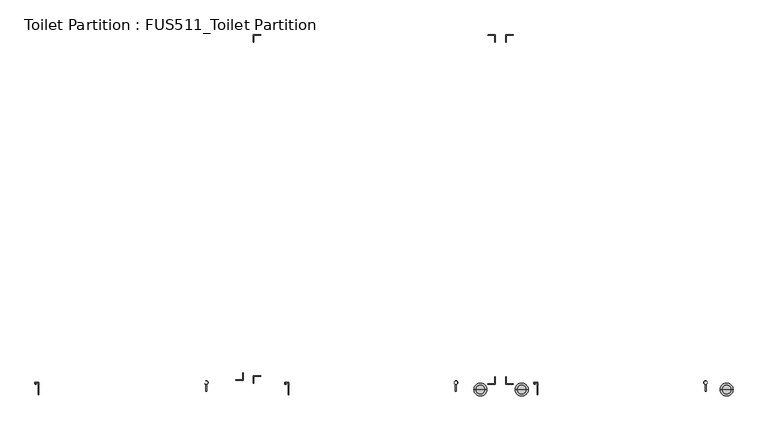
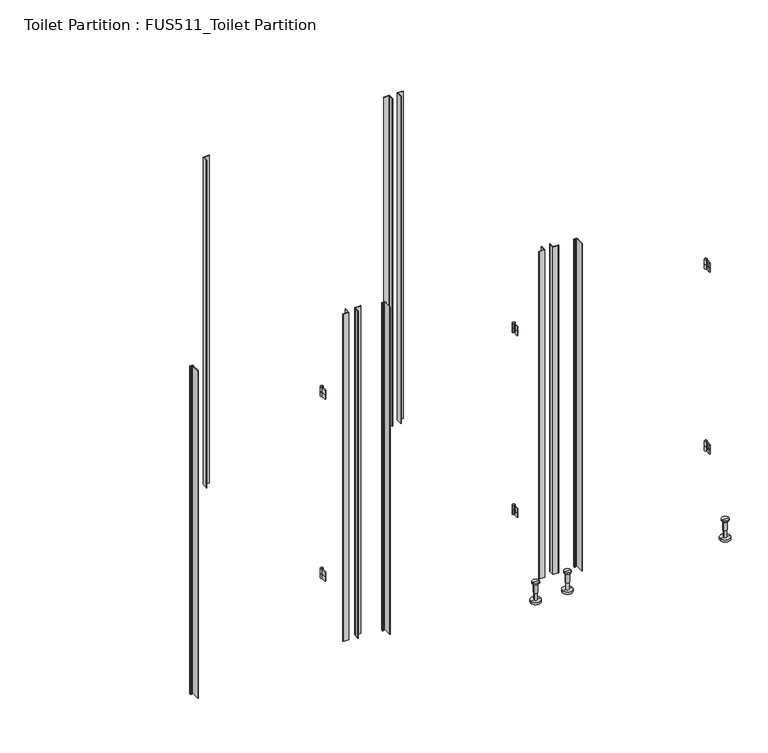
# IFC4 building model written with IfcOpenShell, lengths in millimetres: furniture geometry, Toilet Partition : FUS511_Toilet Partition.
# Revit data of these elements (continued)
# Type "Toilet Partition : FUS511_Toilet Partition"
#   Created by = "Utku Can Kocadağ"
#   Controlled by = "Sefer Özdoğan"
#   Approved by = "Aydın Altınova"
#   Cubicle_Height = 1800 mm
#   Bot_Gap = 100 mm
#   Default Elevation = 0
# Element 1 (IfcFurniture, "Toilet Partition : FUS511_Toilet Partition")
#   Materials on its faces: "Aln_Aluminum_02"
# Materials
#   "Aln_Aluminum_02": class "Generic", colour RGB 120 120 120, transparency 0, Cost = 0
